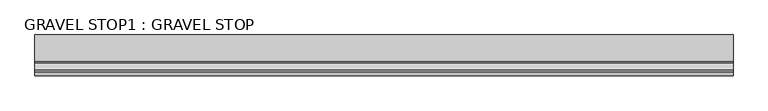
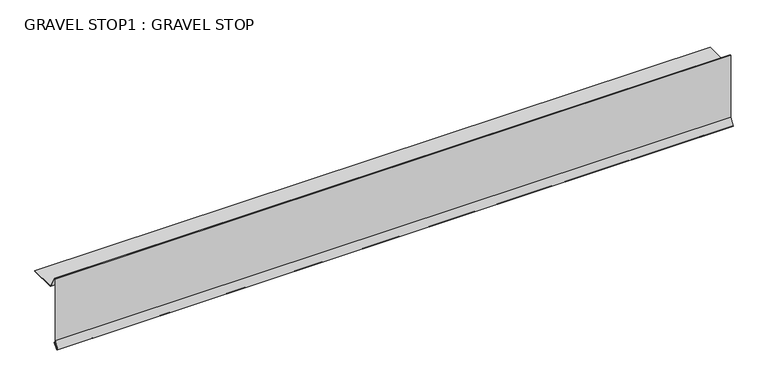
"""IFC4 building model written with IfcOpenShell, lengths in millimetres: proxy geometry, GRAVEL STOP1 : GRAVEL STOP."""

from ifc_helpers import new_model, si_unit, frame, origin, place, context, project, spatial, polyline, outline, extrude, source, transform, mapped, element, save


def gravel_stop1_gravel_stop_d8bdad0e(model_context):
    return source(origin(), model_context, "Body", "SweptSolid", [
        extrude(outline(polyline([(-5587.6106629, 40061.0736754), (-5591.684607, 40064.1815506), (-5580.0356381, 40085.5191254), (-5580.0356381, 40278.1940248), (-5577.0037237, 40279.0064238), (-5556.3332702, 40243.204148), (-5552.58096, 40241.0377507), (-5475.1230533, 40241.0377507), (-5475.1230533, 40239.6266397), (-5552.959066, 40239.6266397), (-5557.3662751, 40242.1711431), (-5577.6843899, 40277.3631503), (-5578.6245271, 40277.1112413), (-5578.6245271, 40085.1590213), (-5589.8655469, 40064.5686925), (-5587.7358967, 40062.9440538), (-5574.2139721, 40076.4659785), (-5573.2161659, 40075.4681723), (-5587.6106629, 40061.0736754)])), frame((12382.7678845, 0.0, 0.0), z_axis=(1.0, 0.0, 0.0), x_axis=(0.0, 1.0, 0.0)), (0.0, 0.0, 1.0), 2000.25),
    ])


if __name__ == "__main__":
    model = new_model("IFC4")
    model_context = context("Model", 3, world=origin())
    ifc_project = project(units=[si_unit("LENGTHUNIT", "METRE", prefix="MILLI")], contexts=[model_context])
    site = spatial("IfcSite", under=ifc_project)
    building = spatial("IfcBuilding", under=site)
    placement = place(None, origin())
    gravel_stop1_gravel_stop_shape = gravel_stop1_gravel_stop_d8bdad0e(model_context)
    element("IfcBuildingElementProxy", 1, Name="GRAVEL STOP1 : GRAVEL STOP", ObjectType="GRAVEL STOP1 : GRAVEL STOP", at=placement, inside=building, context=model_context, shape_type="MappedRepresentation", body=[
        mapped(gravel_stop1_gravel_stop_shape, transform((0.0, 0.0, 0.0), x_axis=(1.0, 0.0, 0.0), y_axis=(0.0, 1.0, 0.0), z_axis=(0.0, 0.0, 1.0))),
    ])
    save(model, "model.ifc")

# Revit data of these elements
# Type "GRAVEL STOP1 : GRAVEL STOP"
#   NameOverride = "GRAVEL STOP"
# Element 1 (IfcBuildingElementProxy, "GRAVEL STOP1 : GRAVEL STOP")
#   Materials on its faces: "GRAVEL STOP REQUIRED WITH GRAVEL SURFACE SYSTEMS"
# Materials
#   "GRAVEL STOP REQUIRED WITH GRAVEL SURFACE SYSTEMS": class "Unassigned", colour RGB 170 170 127, transparency 0, Cost = 0
